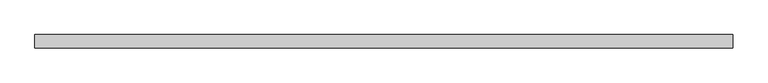
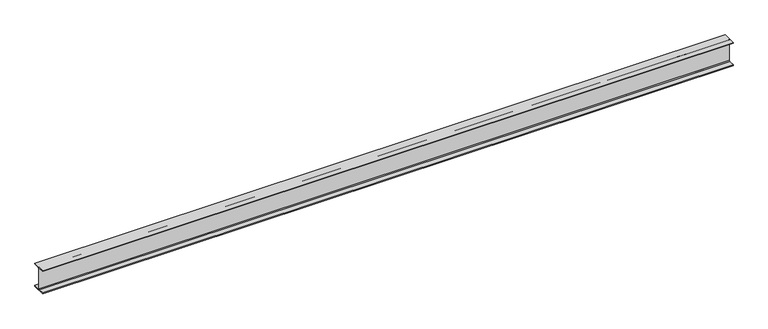
"""IFC4 building model written with IfcOpenShell, lengths in millimetres: beam geometry, Old_Steel Beam_H-KSD3502 : H_SB_ASB_H-300×300x10x15."""

from ifc_helpers import new_model, si_unit, point, frame, frame_2d, origin, place, context, project, spatial, polyline, circle_curve, trimmed, segment, composite_curve, outline, extrude, source, transform, mapped, element, save


def beam_3caf57da(model_context):
    return source(origin(), model_context, "Body", "SweptSolid", [
        extrude(outline(composite_curve([segment(polyline([(82.5, -141.5), (82.5, -151.7), (-82.5, -151.7), (-82.5, -141.5), (-11.9, -141.5)]), True, "CONTINUOUS"), segment(trimmed(circle_curve(frame_2d((-11.9, -132.6)), 8.9), [point((-11.9, -141.5))], [point((-3.0, -132.6))], True, "CARTESIAN"), True, "CONTINUOUS"), segment(polyline([(-3.0, -132.6), (-3.0, 132.6)]), True, "CONTINUOUS"), segment(trimmed(circle_curve(frame_2d((-11.9, 132.6)), 8.9), [point((-3.0, 132.6))], [point((-11.9, 141.5))], True, "CARTESIAN"), True, "CONTINUOUS"), segment(polyline([(-11.9, 141.5), (-82.5, 141.5), (-82.5, 151.7), (82.5, 151.7), (82.5, 141.5), (11.9, 141.5)]), True, "CONTINUOUS"), segment(trimmed(circle_curve(frame_2d((11.9, 132.6)), 8.9), [point((11.9, 141.5))], [point((3.0, 132.6))], True, "CARTESIAN"), True, "CONTINUOUS"), segment(polyline([(3.0, 132.6), (3.0, -132.6)]), True, "CONTINUOUS"), segment(trimmed(circle_curve(frame_2d((11.9, -132.6)), 8.9), [point((3.0, -132.6))], [point((11.9, -141.5))], True, "CARTESIAN"), True, "CONTINUOUS"), segment(polyline([(11.9, -141.5), (82.5, -141.5)]), True, "CONTINUOUS")], self_intersect=False)), frame((-4328.9958952, 0.0, 0.0), z_axis=(1.0, 0.0, 0.0), x_axis=(0.0, 1.0, 0.0)), (0.0, 0.0, 1.0), 8601.9210734),
    ])


if __name__ == "__main__":
    model = new_model("IFC4")
    model_context = context("Model", 3, world=origin())
    ifc_project = project(units=[si_unit("LENGTHUNIT", "METRE", prefix="MILLI")], contexts=[model_context])
    site = spatial("IfcSite", under=ifc_project)
    building = spatial("IfcBuilding", under=site)
    placement = place(None, origin())
    beam_shape = beam_3caf57da(model_context)
    element("IfcBeam", 1, ObjectType="Old_Steel Beam_H-KSD3502 : H_SB_ASB_H-300×300x10x15", at=placement, inside=building, context=model_context, shape_type="MappedRepresentation", body=[
        mapped(beam_shape, transform((0.0, 0.0, 0.0), x_axis=(1.0, 0.0, 0.0), y_axis=(0.0, 1.0, 0.0), z_axis=(0.0, 0.0, 1.0))),
    ])
    save(model, "model.ifc")

# Revit data of these elements
# Type "Old_Steel Beam_H-KSD3502 : H_SB_ASB_H-300×300x10x15"
#   Width = 30.0 cm
#   Web Thickness = 1.0 cm
#   Web Fillet = 1.8 cm
#   Warping Constant = 1370670.0 cm⁶
#   Torsional Moment of Inertia = 77.00 cm⁴
#   Torsional Modulus = 1.0 cm³
#   Section Area = 119.8 cm²
#   Plastic Modulus weak axis = 684.0 cm³
#   Plastic Modulus strong axis = 1500.0 cm³
#   Perimeter = 1.75 m²/m
#   Nominal Weight = 94.00 kgf/m
#   Moment of Inertia weak axis = 6750.00 cm⁴
#   Moment of Inertia strong axis = 20400.00 cm⁴
#   Height = 30.0 cm
#   Flange Thickness = 1.5 cm
#   Elastic Modulus weak axis = 450.0 cm³
#   Elastic Modulus strong axis = 1360.0 cm³
#   Centroid Vertical = 15.0 cm
#   Centroid Horizontal = 15.0 cm
#   Length [instance default] = 1.5240 m
#   Structural Material [instance default] = Steel, 45-345
#   Assembly Code = ""
# Element 1 (IfcBeam, "Old_Steel Beam_H-KSD3502 : H_SB_ASB_H-300×300x10x15")
#   Structural Material = none
# Materials
#   "Steel, 45-345": class "Metal", colour RGB 189 187 185, transparency 0, Description = "Steel 345 MPa", Cost = 0
